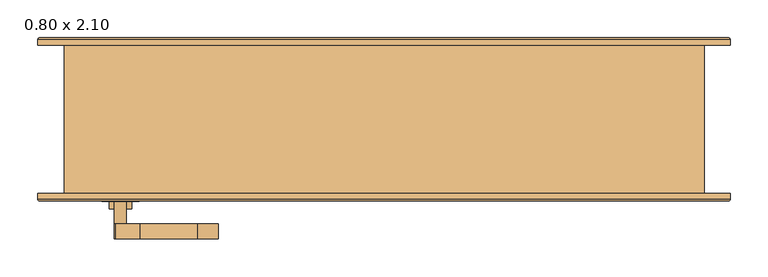
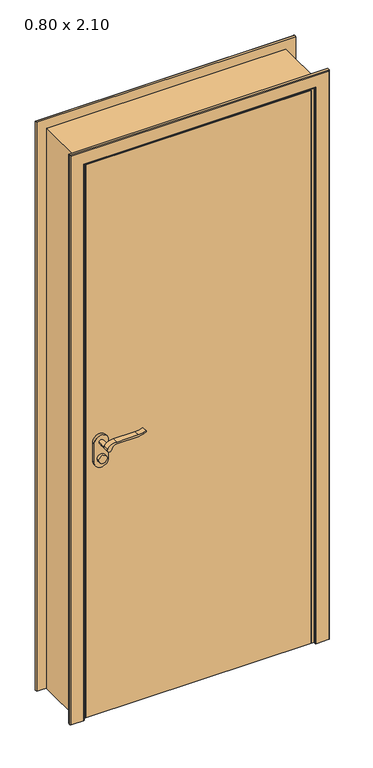
"""IFC4 building model written with IfcOpenShell, lengths in millimetres: door geometry, .CC_ND 300_PORTA SIMPLES DE ABRIR_COM EXTENSÃO : 0.80 x 2.10."""

from ifc_helpers import new_model, si_unit, point, frame, frame_2d, origin, origin_with_axes, place, context, project, spatial, polyline, circle_curve, ellipse_curve, trimmed, segment, composite_curve, outline, extrude, faceted_brep, source, transform, mapped, element, save
from ifc_brep_helpers import plane_surface, cylinder_surface, advanced_brep


def door_0_80_x_2_10_a85ccb46(model_context):
    return source(origin(), model_context, "Body", "SolidModel", [
        extrude(outline(composite_curve([segment(trimmed(circle_curve(frame_2d((964.5, -350.0)), 15.0), [point((964.5, -335.0))], [point((964.5, -365.0))], False, "CARTESIAN"), True, "CONTINUOUS"), segment(trimmed(circle_curve(frame_2d((964.5, -350.0)), 15.0), [point((964.5, -365.0))], [point((964.5, -335.0))], False, "CARTESIAN"), True, "CONTINUOUS")], self_intersect=False)), frame((0.0, -118.8, 0.0), z_axis=(0.0, 1.0, 0.0), x_axis=(0.0, 0.0, 1.0)), (0.0, 0.0, 1.0), 10.0),
        extrude(outline(composite_curve([segment(trimmed(circle_curve(frame_2d((964.5, -350.0)), 15.0), [point((964.5, -335.0))], [point((964.5, -365.0))], False, "CARTESIAN"), True, "CONTINUOUS"), segment(trimmed(circle_curve(frame_2d((964.5, -350.0)), 15.0), [point((964.5, -365.0))], [point((964.5, -335.0))], False, "CARTESIAN"), True, "CONTINUOUS")], self_intersect=False)), frame((0.0, -58.8, 0.0), z_axis=(0.0, 1.0, 0.0), x_axis=(0.0, 0.0, 1.0)), (0.0, 0.0, 1.0), 10.0),
        extrude(outline(composite_curve([segment(trimmed(circle_curve(frame_2d((1024.5, -350.0)), 8.0), [point((1029.1523287, -356.5081363))], [point((1024.5, -342.0))], False, "CARTESIAN"), True, "CONTINUOUS"), segment(trimmed(circle_curve(frame_2d((1019.3738613, -324.6138099)), 18.1261387), [point((1024.5, -342.0))], [point((1037.5, -324.6138099))], True, "CARTESIAN"), True, "CONTINUOUS"), segment(polyline([(1037.5, -324.6138099), (1037.5, -248.3564091)]), True, "CONTINUOUS"), segment(trimmed(circle_curve(frame_2d((1096.7709207, -251.9396612)), 59.3791355), [point((1037.5, -248.3564091))], [point((1046.7135558, -220.0))], False, "CARTESIAN"), True, "CONTINUOUS"), segment(polyline([(1046.7135558, -220.0), (1049.5, -220.0)]), True, "CONTINUOUS"), segment(trimmed(circle_curve(frame_2d((1127.7850638, -248.4227909)), 83.2850902), [point((1049.5, -220.0))], [point((1044.5, -248.3564091))], True, "CARTESIAN"), True, "CONTINUOUS"), segment(polyline([(1044.5, -248.3564091), (1044.5, -324.6325667)]), True, "CONTINUOUS"), segment(trimmed(circle_curve(frame_2d((1007.2555521, -326.3324871)), 37.2832219), [point((1044.5, -324.6325667))], [point((1029.1523287, -356.5081363))], False, "CARTESIAN"), True, "CONTINUOUS")], self_intersect=False)), frame((0.0, -158.8, 0.0), z_axis=(0.0, 1.0, 0.0), x_axis=(0.0, 0.0, 1.0)), (0.0, 0.0, 1.0), 20.0),
        extrude(outline(composite_curve([segment(trimmed(circle_curve(frame_2d((1019.3738682, -324.6138122)), 18.1261318), [point((1024.4999903, -342.0))], [point((1037.5, -324.6138122))], True, "CARTESIAN"), True, "CONTINUOUS"), segment(polyline([(1037.5, -324.6138122), (1037.5, -248.3564091)]), True, "CONTINUOUS"), segment(trimmed(circle_curve(frame_2d((1096.7709207, -251.9396612)), 59.3791355), [point((1037.5, -248.3564091))], [point((1046.7135558, -220.0))], False, "CARTESIAN"), True, "CONTINUOUS"), segment(polyline([(1046.7135558, -220.0), (1049.5, -220.0)]), True, "CONTINUOUS"), segment(trimmed(circle_curve(frame_2d((1127.7850638, -248.4227909)), 83.2850902), [point((1049.5, -220.0))], [point((1044.5, -248.3564091))], True, "CARTESIAN"), True, "CONTINUOUS"), segment(polyline([(1044.5, -248.3564091), (1044.5, -324.6325667)]), True, "CONTINUOUS"), segment(trimmed(circle_curve(frame_2d((1007.2555521, -326.3324871)), 37.2832219), [point((1044.5, -324.6325667))], [point((1029.1523287, -356.5081363))], False, "CARTESIAN"), True, "CONTINUOUS"), segment(trimmed(circle_curve(frame_2d((1024.5, -350.0)), 8.0), [point((1029.1523287, -356.5081363))], [point((1024.4999903, -342.0))], False, "CARTESIAN"), True, "CONTINUOUS")], self_intersect=False)), frame((0.0, -28.8, 0.0), z_axis=(0.0, 1.0, 0.0), x_axis=(0.0, 0.0, 1.0)), (0.0, 0.0, 1.0), 20.0),
        extrude(outline(composite_curve([segment(trimmed(circle_curve(frame_2d((1024.5, -350.0)), 8.0), [point((1024.5, -342.0))], [point((1024.5, -358.0))], False, "CARTESIAN"), True, "CONTINUOUS"), segment(trimmed(circle_curve(frame_2d((1024.5, -350.0)), 8.0), [point((1024.5, -358.0))], [point((1024.5, -342.0))], False, "CARTESIAN"), True, "CONTINUOUS")], self_intersect=False)), frame((0.0, -138.8, 0.0), z_axis=(0.0, 1.0, 0.0), x_axis=(0.0, 0.0, 1.0)), (0.0, 0.0, 1.0), 30.0),
        extrude(outline(composite_curve([segment(trimmed(circle_curve(frame_2d((1024.5, -350.0)), 8.0), [point((1024.5, -342.0))], [point((1024.5, -358.0))], False, "CARTESIAN"), True, "CONTINUOUS"), segment(trimmed(circle_curve(frame_2d((1024.5, -350.0)), 8.0), [point((1024.5, -358.0))], [point((1024.5, -342.0))], False, "CARTESIAN"), True, "CONTINUOUS")], self_intersect=False)), frame((0.0, -58.8, 0.0), z_axis=(0.0, 1.0, 0.0), x_axis=(0.0, 0.0, 1.0)), (0.0, 0.0, 1.0), 30.0),
        extrude(outline(composite_curve([segment(trimmed(circle_curve(frame_2d((954.5, -350.0)), 25.0), [point((954.5, -375.0))], [point((954.5, -325.0))], False, "CARTESIAN"), True, "CONTINUOUS"), segment(polyline([(954.5, -325.0), (1024.5, -325.0)]), True, "CONTINUOUS"), segment(trimmed(circle_curve(frame_2d((1024.5, -350.0)), 25.0), [point((1024.5, -325.0))], [point((1024.5, -375.0))], False, "CARTESIAN"), True, "CONTINUOUS"), segment(polyline([(1024.5, -375.0), (954.5, -375.0)]), True, "CONTINUOUS")], self_intersect=False)), frame((0.0, -108.8, 0.0), z_axis=(0.0, 1.0, 0.0), x_axis=(0.0, 0.0, 1.0)), (0.0, 0.0, 1.0), 10.0),
        extrude(outline(composite_curve([segment(trimmed(circle_curve(frame_2d((954.5, -350.0)), 25.0), [point((954.5, -375.0))], [point((954.5, -325.0))], False, "CARTESIAN"), True, "CONTINUOUS"), segment(polyline([(954.5, -325.0), (1024.5, -325.0)]), True, "CONTINUOUS"), segment(trimmed(circle_curve(frame_2d((1024.5, -350.0)), 25.0), [point((1024.5, -325.0))], [point((1024.5, -375.0))], False, "CARTESIAN"), True, "CONTINUOUS"), segment(polyline([(1024.5, -375.0), (954.5, -375.0)]), True, "CONTINUOUS")], self_intersect=False)), frame((0.0, -68.8, 0.0), z_axis=(0.0, 1.0, 0.0), x_axis=(0.0, 0.0, 1.0)), (0.0, 0.0, 1.0), 10.0),
        faceted_brep([(392.0, 98.8, 0.0), (425.0, 98.8, 0.0), (425.0, -98.8, 0.0), (400.0, -98.8, 0.0), (400.0, -68.8, 0.0), (392.0, -68.8, 0.0), (392.0, 98.8, 2067.0), (-392.0, 98.8, 2067.0), (-392.0, 98.8, 0.0), (-425.0, 98.8, 0.0), (-425.0, 98.8, 2100.0), (425.0, 98.8, 2100.0), (425.0, -98.8, 2100.0), (-425.0, -98.8, 2100.0), (-425.0, -98.8, 0.0), (-400.0, -98.8, 0.0), (-400.0, -98.8, 2075.0), (400.0, -98.8, 2075.0), (400.0, -68.8, 2075.0), (-400.0, -68.8, 2075.0), (-400.0, -68.8, 0.0), (-392.0, -68.8, 0.0), (-392.0, -68.8, 2067.0), (392.0, -68.8, 2067.0)], [[[0, 1, 2, 3, 4, 5]], [[1, 0, 6, 7, 8, 9, 10, 11]], [[2, 1, 11, 12]], [[3, 2, 12, 13, 14, 15, 16, 17]], [[4, 3, 17, 18]], [[5, 4, 18, 19, 20, 21, 22, 23]], [[0, 5, 23, 6]], [[7, 22, 21, 8]], [[8, 21, 20, 15, 14, 9]], [[13, 10, 9, 14]], [[19, 16, 15, 20]], [[12, 11, 10, 13]], [[18, 17, 16, 19]], [[6, 23, 22, 7]]]),
        extrude(outline(polyline([(-400.0, -68.8), (400.0, -68.8), (400.0, -98.8), (-400.0, -98.8), (-400.0, -68.8)])), origin_with_axes(), (0.0, 0.0, 1.0), 2075.0),
        advanced_brep(
        [(-460.0, -98.8, 0.0), (-410.0, -98.8, 0.0), (-410.0, -105.8, 0.0), (-413.0, -108.8, 0.0), (-457.0, -108.8, 0.0), (-460.0, -105.8, 0.0), (-460.0, -98.8, 2135.0), (460.0, -98.8, 2135.0), (460.0, -98.8, 0.0), (410.0, -98.8, 0.0), (410.0, -98.8, 2085.0), (-410.0, -98.8, 2085.0), (-410.0, -105.8, 2085.0), (-413.0, -108.8, 2088.0), (413.0, -108.8, 2088.0), (413.0, -108.8, 0.0), (457.0, -108.8, 0.0), (457.0, -108.8, 2132.0), (-457.0, -108.8, 2132.0), (-460.0, -105.8, 2135.0), (460.0, -105.8, 2135.0), (460.0, -105.8, 0.0), (410.0, -105.8, 0.0), (410.0, -105.8, 2085.0)],
        [
            (0, 1),
            (1, 2),
            (2, 3, circle_curve(frame((-413.0, -105.8, 0.0), z_axis=(0.0, 0.0, -1.0), x_axis=(1.0, 0.0, 0.0)), 3.0)),
            (3, 4),
            (4, 5, circle_curve(frame((-457.0, -105.8, 0.0), z_axis=(0.0, 0.0, -1.0), x_axis=(1.0, 0.0, 0.0)), 3.0)),
            (5, 0),
            (0, 6),
            (6, 7),
            (7, 8),
            (8, 9),
            (9, 10),
            (10, 11),
            (11, 1),
            (11, 12),
            (12, 2),
            (12, 13, ellipse_curve(frame((-413.0, -105.8, 2088.0), z_axis=(-0.7071067811865475, 0.0, -0.7071067811865475), x_axis=(0.7071067811865474, 0.0, -0.7071067811865476)), 4.2426407, 3.0)),
            (13, 3),
            (13, 14),
            (14, 15),
            (15, 16),
            (16, 17),
            (17, 18),
            (18, 4),
            (18, 19, ellipse_curve(frame((-457.0, -105.8, 2132.0), z_axis=(-0.7071067811865475, 0.0, -0.7071067811865475), x_axis=(0.7071067811865474, 0.0, -0.7071067811865476)), 4.2426407, 3.0)),
            (19, 5),
            (19, 6),
            (7, 20),
            (20, 21),
            (21, 8),
            (21, 16, circle_curve(frame((457.0, -105.8, 0.0), z_axis=(0.0, 0.0, -1.0), x_axis=(-1.0, 0.0, 0.0)), 3.0)),
            (15, 22, circle_curve(frame((413.0, -105.8, 0.0), z_axis=(0.0, 0.0, -1.0), x_axis=(-1.0, 0.0, 0.0)), 3.0)),
            (22, 9),
            (23, 10),
            (22, 23),
            (14, 23, ellipse_curve(frame((413.0, -105.8, 2088.0), z_axis=(0.7071067811865475, 0.0, -0.7071067811865475), x_axis=(0.7071067811865474, 0.0, 0.7071067811865476)), 4.2426407, 3.0)),
            (20, 17, ellipse_curve(frame((457.0, -105.8, 2132.0), z_axis=(0.7071067811865475, 0.0, -0.7071067811865475), x_axis=(0.7071067811865474, 0.0, 0.7071067811865476)), 4.2426407, 3.0)),
            (23, 12),
            (19, 20),
        ],
        [
            plane_surface(frame((-410.0, -98.8, 0.0), z_axis=(0.0, 0.0, -1.0), x_axis=(0.0, 1.0, 0.0))),
            plane_surface(frame((-460.0, -98.8, 0.0), z_axis=(0.0, 1.0, 0.0), x_axis=(0.0, 0.0, 1.0))),
            plane_surface(frame((-410.0, -98.8, 0.0), z_axis=(1.0, 0.0, 0.0), x_axis=(0.0, 0.0, 1.0))),
            cylinder_surface(frame((-413.0, -105.8, 0.0), z_axis=(0.0, 0.0, -1.0), x_axis=(1.0, 0.0, 0.0)), 3.0),
            plane_surface(frame((-413.0, -108.8, 0.0), z_axis=(0.0, -1.0, 0.0), x_axis=(0.0, 0.0, 1.0))),
            cylinder_surface(frame((-457.0, -105.8, 0.0), z_axis=(0.0, 0.0, -1.0), x_axis=(1.0, 0.0, 0.0)), 3.0),
            plane_surface(frame((-460.0, -105.8, 0.0), z_axis=(-1.0, 0.0, 0.0), x_axis=(0.0, 0.0, 1.0))),
            plane_surface(frame((460.0, -105.8, 2135.0), z_axis=(1.0, 0.0, 0.0), x_axis=(0.0, 0.0, -1.0))),
            plane_surface(frame((410.0, -98.8, 0.0), z_axis=(0.0, 0.0, -1.0), x_axis=(0.0, 1.0, 0.0))),
            plane_surface(frame((410.0, -98.8, 2085.0), z_axis=(-1.0, 0.0, 0.0), x_axis=(0.0, 0.0, -1.0))),
            cylinder_surface(frame((413.0, -105.8, 2085.0), z_axis=(0.0, 0.0, 1.0), x_axis=(-1.0, 0.0, 0.0)), 3.0),
            cylinder_surface(frame((457.0, -105.8, 2085.0), z_axis=(0.0, 0.0, 1.0), x_axis=(-1.0, 0.0, 0.0)), 3.0),
            plane_surface(frame((-410.0, -98.8, 2085.0), z_axis=(0.0, 0.0, -1.0), x_axis=(1.0, 0.0, 0.0))),
            plane_surface(frame((-460.0, -105.8, 2135.0), z_axis=(0.0, 0.0, 1.0), x_axis=(1.0, 0.0, 0.0))),
            cylinder_surface(frame((-410.0, -105.8, 2088.0), z_axis=(-1.0, 0.0, 0.0), x_axis=(0.0, 0.0, -1.0)), 3.0),
            cylinder_surface(frame((-410.0, -105.8, 2132.0), z_axis=(-1.0, 0.0, 0.0), x_axis=(0.0, 0.0, -1.0)), 3.0),
        ],
        [
            (0, [[1, 2, 3, 4, 5, 6]]),
            (1, [[-1, 7, 8, 9, 10, 11, 12, 13]]),
            (2, [[-2, -13, 14, 15]]),
            (3, [[-3, -15, 16, 17]]),
            (4, [[-4, -17, 18, 19, 20, 21, 22, 23]]),
            (5, [[-5, -23, 24, 25]]),
            (6, [[-6, -25, 26, -7]]),
            (7, [[27, 28, 29, -9]]),
            (8, [[-29, 30, -20, 31, 32, -10]]),
            (9, [[33, -11, -32, 34]]),
            (10, [[35, -34, -31, -19]]),
            (11, [[36, -21, -30, -28]]),
            (12, [[-14, -12, -33, 37]]),
            (13, [[-26, 38, -27, -8]]),
            (14, [[-16, -37, -35, -18]]),
            (15, [[-24, -22, -36, -38]]),
        ],
    ),
        advanced_brep(
        [(460.0, 98.8, 0.0), (410.0, 98.8, 0.0), (410.0, 105.8157283, 0.0), (412.9842717, 108.8, 0.0), (457.0342217, 108.8, 0.0), (460.0, 105.8342217, 0.0), (460.0, 98.8, 2135.0), (-460.0, 98.8, 2135.0), (-460.0, 98.8, 0.0), (-410.0, 98.8, 0.0), (-410.0, 98.8, 2085.0), (410.0, 98.8, 2085.0), (410.0, 105.8157283, 2085.0), (412.9842717, 108.8, 2087.9842717), (-412.9842717, 108.8, 2087.9842717), (-412.9842717, 108.8, 0.0), (-457.0342217, 108.8, 0.0), (-457.0342217, 108.8, 2132.0342217), (457.0342217, 108.8, 2132.0342217), (460.0, 105.8342217, 2135.0), (-460.0, 105.8342217, 2135.0), (-460.0, 105.8342217, 0.0), (-410.0, 105.8157283, 0.0), (-410.0, 105.8157283, 2085.0)],
        [
            (0, 1),
            (1, 2),
            (2, 3, circle_curve(frame((412.9842717, 105.8157283, 0.0), z_axis=(0.0, 0.0, -1.0), x_axis=(1.0, 0.0, 0.0)), 2.9842717)),
            (3, 4),
            (4, 5, circle_curve(frame((457.0342217, 105.8342217, 0.0), z_axis=(0.0, 0.0, -1.0), x_axis=(1.0, 0.0, 0.0)), 2.9657783)),
            (5, 0),
            (0, 6),
            (6, 7),
            (7, 8),
            (8, 9),
            (9, 10),
            (10, 11),
            (11, 1),
            (11, 12),
            (12, 2),
            (12, 13, ellipse_curve(frame((412.9842717, 105.8157283, 2087.9842717), z_axis=(0.7071067811865475, 0.0, -0.7071067811865475), x_axis=(-0.7071067811865474, 0.0, -0.7071067811865476)), 4.2203975, 2.9842717)),
            (13, 3),
            (13, 14),
            (14, 15),
            (15, 16),
            (16, 17),
            (17, 18),
            (18, 4),
            (18, 19, ellipse_curve(frame((457.0342217, 105.8342217, 2132.0342217), z_axis=(0.7071067811865475, 0.0, -0.7071067811865475), x_axis=(-0.7071067811865474, 0.0, -0.7071067811865476)), 4.1942438, 2.9657783)),
            (19, 5),
            (19, 6),
            (7, 20),
            (20, 21),
            (21, 8),
            (21, 16, circle_curve(frame((-457.0342217, 105.8342217, 0.0), z_axis=(0.0, 0.0, -1.0), x_axis=(-1.0, 0.0, 0.0)), 2.9657783)),
            (15, 22, circle_curve(frame((-412.9842717, 105.8157283, 0.0), z_axis=(0.0, 0.0, -1.0), x_axis=(-1.0, 0.0, 0.0)), 2.9842717)),
            (22, 9),
            (23, 10),
            (22, 23),
            (14, 23, ellipse_curve(frame((-412.9842717, 105.8157283, 2087.9842717), z_axis=(-0.7071067811865475, 0.0, -0.7071067811865475), x_axis=(-0.7071067811865474, 0.0, 0.7071067811865476)), 4.2203975, 2.9842717)),
            (20, 17, ellipse_curve(frame((-457.0342217, 105.8342217, 2132.0342217), z_axis=(-0.7071067811865475, 0.0, -0.7071067811865475), x_axis=(-0.7071067811865474, 0.0, 0.7071067811865476)), 4.1942438, 2.9657783)),
            (23, 12),
            (19, 20),
        ],
        [
            plane_surface(frame((410.0, 98.8, 0.0), z_axis=(0.0, 0.0, -1.0), x_axis=(0.0, 1.0, 0.0))),
            plane_surface(frame((460.0, 98.8, 0.0), z_axis=(0.0, -1.0, 0.0), x_axis=(0.0, 0.0, 1.0))),
            plane_surface(frame((410.0, 98.8, 0.0), z_axis=(-1.0, 0.0, 0.0), x_axis=(0.0, 0.0, 1.0))),
            cylinder_surface(frame((412.9842717, 105.8157283, 0.0), z_axis=(0.0, 0.0, -1.0), x_axis=(1.0, 0.0, 0.0)), 2.9842717),
            plane_surface(frame((412.9842717, 108.8, 0.0), z_axis=(0.0, 1.0, 0.0), x_axis=(0.0, 0.0, 1.0))),
            cylinder_surface(frame((457.0342217, 105.8342217, 0.0), z_axis=(0.0, 0.0, -1.0), x_axis=(1.0, 0.0, 0.0)), 2.9657783),
            plane_surface(frame((460.0, 105.8342217, 0.0), z_axis=(1.0, 0.0, 0.0), x_axis=(0.0, 0.0, 1.0))),
            plane_surface(frame((-460.0, 105.8342217, 2135.0), z_axis=(-1.0, 0.0, 0.0), x_axis=(0.0, 0.0, -1.0))),
            plane_surface(frame((-410.0, 98.8, 0.0), z_axis=(0.0, 0.0, -1.0), x_axis=(0.0, 1.0, 0.0))),
            plane_surface(frame((-410.0, 98.8, 2085.0), z_axis=(1.0, 0.0, 0.0), x_axis=(0.0, 0.0, -1.0))),
            cylinder_surface(frame((-412.9842717, 105.8157283, 2085.0), z_axis=(0.0, 0.0, 1.0), x_axis=(-1.0, 0.0, 0.0)), 2.9842717),
            cylinder_surface(frame((-457.0342217, 105.8342217, 2085.0), z_axis=(0.0, 0.0, 1.0), x_axis=(-1.0, 0.0, 0.0)), 2.9657783),
            plane_surface(frame((410.0, 98.8, 2085.0), z_axis=(0.0, 0.0, -1.0), x_axis=(-1.0, 0.0, 0.0))),
            plane_surface(frame((460.0, 105.8342217, 2135.0), z_axis=(0.0, 0.0, 1.0), x_axis=(-1.0, 0.0, 0.0))),
            cylinder_surface(frame((410.0, 105.8157283, 2087.9842717), z_axis=(1.0, 0.0, 0.0), x_axis=(0.0, 0.0, 1.0)), 2.9842717),
            cylinder_surface(frame((410.0, 105.8342217, 2132.0342217), z_axis=(1.0, 0.0, 0.0), x_axis=(0.0, 0.0, 1.0)), 2.9657783),
        ],
        [
            (0, [[1, 2, 3, 4, 5, 6]]),
            (1, [[-1, 7, 8, 9, 10, 11, 12, 13]]),
            (2, [[-2, -13, 14, 15]]),
            (3, [[-3, -15, 16, 17]]),
            (4, [[-4, -17, 18, 19, 20, 21, 22, 23]]),
            (5, [[-5, -23, 24, 25]]),
            (6, [[-6, -25, 26, -7]]),
            (7, [[27, 28, 29, -9]]),
            (8, [[-29, 30, -20, 31, 32, -10]]),
            (9, [[33, -11, -32, 34]]),
            (10, [[35, -34, -31, -19]]),
            (11, [[36, -21, -30, -28]]),
            (12, [[-14, -12, -33, 37]]),
            (13, [[-26, 38, -27, -8]]),
            (14, [[-16, -37, -35, -18]]),
            (15, [[-24, -22, -36, -38]]),
        ],
    ),
    ])


if __name__ == "__main__":
    model = new_model("IFC4")
    model_context = context("Model", 3, world=origin())
    ifc_project = project(units=[si_unit("LENGTHUNIT", "METRE", prefix="MILLI")], contexts=[model_context])
    site = spatial("IfcSite", under=ifc_project)
    building = spatial("IfcBuilding", under=site)
    placement = place(None, origin())
    door_0_80_x_2_10_shape = door_0_80_x_2_10_a85ccb46(model_context)
    element("IfcDoor", 1, ObjectType=".CC_ND 300_PORTA SIMPLES DE ABRIR_COM EXTENSÃO : 0.80 x 2.10", at=placement, inside=building, context=model_context, shape_type="MappedRepresentation", body=[
        mapped(door_0_80_x_2_10_shape, transform((0.0, 0.0, 0.0), x_axis=(1.0, 0.0, 0.0), y_axis=(0.0, 1.0, 0.0), z_axis=(0.0, 0.0, 1.0))),
    ])
    save(model, "model.ifc")

# Revit data of these elements
# Type ".CC_ND 300_PORTA SIMPLES DE ABRIR_COM EXTENSÃO : 0.80 x 2.10"
#   Type Mark = "153"
#   Analytic Construction = "<None>"
#   Rough Width = 0.85 m
#   Espessura moldura externa = 0.01 m
#   Espessura moldura interna = 0.01 m
#   Largura moldura = 0.05 m
#   Extensão acabamento exterior [instance default] = 0.00 m
#   Extensão acabamento interior [instance default] = 0.00 m
#   Espessura batente = 0.025 m
#   Thickness = 0.03 m
#   Altura batente = 2.085 m
#   Aux Arco [instance default] = 0.80 m
#   Rough Height = 2.125 m
#   Height = 2.10 m
#   Width = 0.80 m
#   Moldura interna [instance default] = yes
#   Moldura externa [instance default] = yes
#   Porta = .MADEIRA COM PINTURA ESMALTE BRANCO ACETINADO
#   Moldura = .MADEIRA COM PINTURA ESMALTE BRANCO ACETINADO
#   Maçaneta = .ALUMÍNIO
#   Batente = .MADEIRA COM PINTURA ESMALTE BRANCO ACETINADO
#   Function = (empty or 0)
#   Wall Closure = (empty or 0)
# Element 1 (IfcDoor, ".CC_ND 300_PORTA SIMPLES DE ABRIR_COM EXTENSÃO : 0.80 x 2.10")
#   Materials on its faces: ".MADEIRA COM PINTURA ESMALTE BRANCO ACETINADO", ".ALUMÍNIO"
# Materials
#   ".MADEIRA COM PINTURA ESMALTE BRANCO ACETINADO": class ".CC_MADEIRAS", colour RGB 240 240 240, transparency 0, Description = "Madeira com pintura esmalte branco acetinado.", Cost = 0
#   ".ALUMÍNIO": class "CC_METAIS", colour RGB 244 244 244, transparency 0, Description = "Material alumínio", Cost = 0
